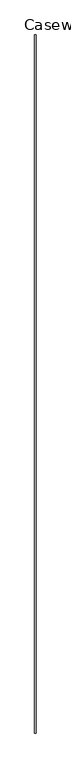
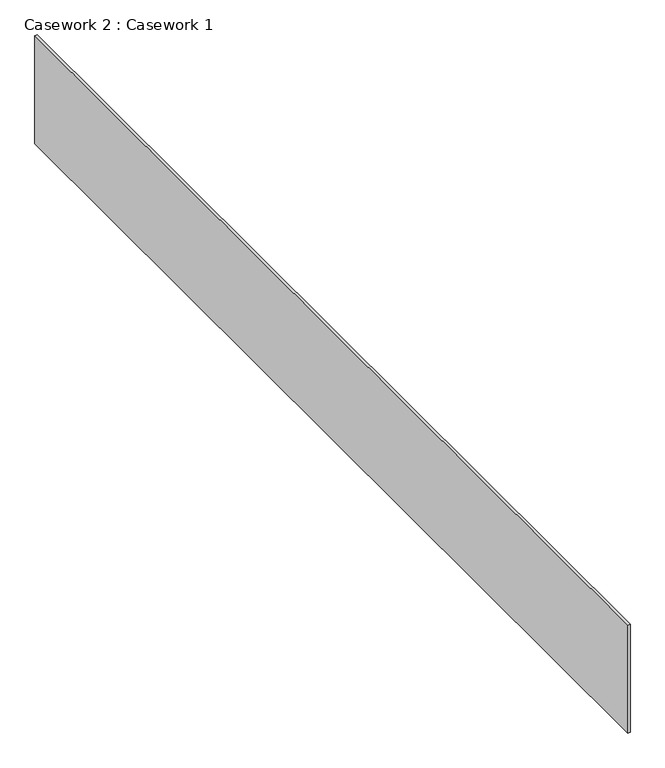
"""IFC4 building model written with IfcOpenShell, lengths in millimetres: furniture geometry, Casework 2 : Casework 1."""

from ifc_helpers import new_model, si_unit, frame, origin, place, context, project, spatial, polyline, outline, extrude, source, transform, mapped, element, save


def casework_2_casework_1_ca6f7087(model_context):
    return source(origin(), model_context, "Body", "SweptSolid", [
        extrude(outline(polyline([(-58955.4926606, 273663.2347125), (-58955.4926606, 285406.6602108), (-58930.0926606, 285406.6602108), (-58930.0926606, 273663.2347125), (-58955.4926606, 273663.2347125)])), frame((0.0, 0.0, 3340.1), z_axis=(0.0, 0.0, 1.0), x_axis=(1.0, 0.0, 0.0)), (0.0, 0.0, 1.0), 1303.445648),
    ])


if __name__ == "__main__":
    model = new_model("IFC4")
    model_context = context("Model", 3, world=origin())
    ifc_project = project(units=[si_unit("LENGTHUNIT", "METRE", prefix="MILLI")], contexts=[model_context])
    site = spatial("IfcSite", under=ifc_project)
    building = spatial("IfcBuilding", under=site)
    placement = place(None, origin())
    casework_2_casework_1_shape = casework_2_casework_1_ca6f7087(model_context)
    element("IfcFurniture", 1, ObjectType="Casework 2 : Casework 1", at=placement, inside=building, context=model_context, shape_type="MappedRepresentation", body=[
        mapped(casework_2_casework_1_shape, transform((0.0, 0.0, 0.0), x_axis=(1.0, 0.0, 0.0), y_axis=(0.0, 1.0, 0.0), z_axis=(0.0, 0.0, 1.0))),
    ])
    save(model, "model.ifc")

# Revit data of these elements
# Element 1 (IfcFurniture, "Casework 2 : Casework 1")
#   Materials on its faces: "METAL PANEL (DARK BRONZE) - TO MATCH MAIN BUILDING ACCENT METAL"
# Materials
#   "METAL PANEL (DARK BRONZE) - TO MATCH MAIN BUILDING ACCENT METAL": class "Generic", colour RGB 88 62 61, transparency 0, Cost = 0
